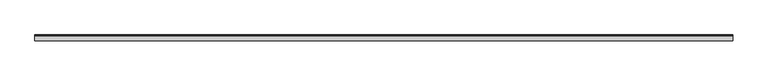
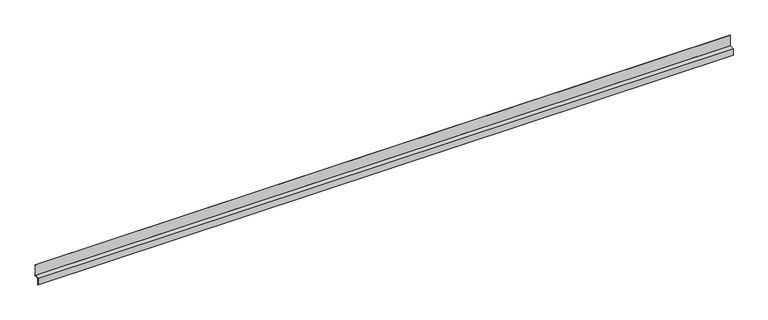
"""IFC4 building model written with IfcOpenShell, lengths in millimetres: proxy geometry, Footer2:Footer002:287073 : Footer2:Footer002:287073."""

from ifc_helpers import new_model, si_unit, frame, origin, place, context, project, spatial, polyline, outline, extrude, source, transform, mapped, element, save


def generic_models_0b863fc5(model_context):
    return source(origin(), model_context, "Body", "SweptSolid", [
        extrude(outline(polyline([(-3970.5899957, 40169.896), (-3970.5899957, 40150.796), (-3971.8599957, 40150.796), (-3971.8599957, 40171.166), (-3957.5717561, 40171.166), (-3957.5717561, 40202.916), (-3956.3017561, 40202.916), (-3956.3017561, 40171.166), (-3955.491909, 40171.166), (-3955.491909, 40169.896), (-3970.5899957, 40169.896)])), frame((17160.0269925, 0.0, 0.0), z_axis=(1.0, 0.0, 0.0), x_axis=(0.0, 1.0, 0.0)), (0.0, 0.0, 1.0), 2000.0),
    ])


if __name__ == "__main__":
    model = new_model("IFC4")
    model_context = context("Model", 3, world=origin())
    ifc_project = project(units=[si_unit("LENGTHUNIT", "METRE", prefix="MILLI")], contexts=[model_context])
    site = spatial("IfcSite", under=ifc_project)
    building = spatial("IfcBuilding", under=site)
    placement = place(None, origin())
    generic_models_shape = generic_models_0b863fc5(model_context)
    element("IfcBuildingElementProxy", 1, Name="Footer2:Footer002:287073 : Footer2:Footer002:287073", ObjectType="Footer2:Footer002:287073 : Footer2:Footer002:287073", at=placement, inside=building, context=model_context, shape_type="MappedRepresentation", body=[
        mapped(generic_models_shape, transform((0.0, 0.0, 0.0), x_axis=(1.0, 0.0, 0.0), y_axis=(0.0, 1.0, 0.0), z_axis=(0.0, 0.0, 1.0))),
    ])
    save(model, "model.ifc")

# Revit data of these elements
# Type "Footer2:Footer002:287073 : Footer2:Footer002:287073"
#   NameOverride = "Footer2:Footer002:287073"
#   ObjectTypeOverride = "Footer2:Footer002"
#   Reference = "Footer002"
#   Category = "Generic Models"
#   Tag = "287073"
# Element 1 (IfcBuildingElementProxy, "Footer2:Footer002:287073 : Footer2:Footer002:287073")
#   Materials on its faces: "SHADOW Z REVEAL  BEAD"
# Materials
#   "SHADOW Z REVEAL  BEAD": class "Unassigned", colour RGB 251 232 155, transparency 0, Cost = 0
